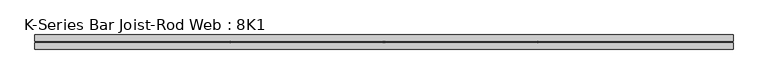
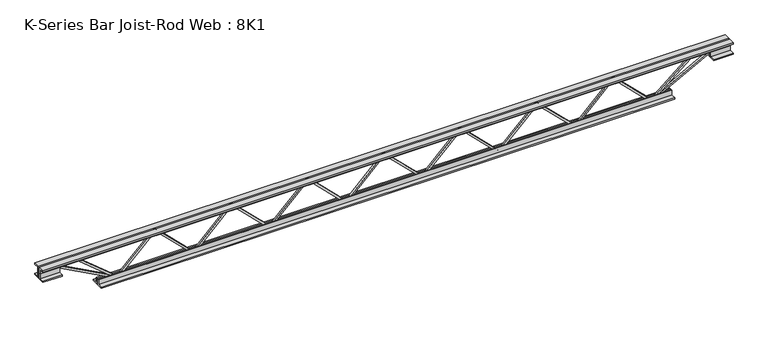
"""IFC4 building model written with IfcOpenShell, lengths in millimetres: beam geometry, K-Series Bar Joist-Rod Web : 8K1."""

from ifc_helpers import new_model, si_unit, frame, origin, place, context, project, spatial, polyline, outline, extrude, source, transform, mapped, element, save


def k_series_bar_joist_rod_web_8k1_41fa30a3(model_context):
    return source(origin(), model_context, "Body", "SweptSolid", [
        extrude(outline(polyline([(-90.4875, 598.572914), (-100.0125, 598.572914), (-100.0125, 603.7011887), (90.4875, 796.8754933), (90.4875, 799.3189439), (-100.0125, 992.4932486), (-100.0125, 997.6215233), (-90.4875, 997.6215233), (-90.4875, 996.399798), (100.0125, 803.2254933), (100.0125, 792.9689439), (-90.4875, 599.7946393), (-90.4875, 598.572914)])), frame((0.0, -4.7625, 0.0), z_axis=(0.0, 1.0, 0.0), x_axis=(0.0, 0.0, 1.0)), (0.0, 0.0, 1.0), 9.525),
        extrude(outline(polyline([(-90.4875, 199.5243047), (-100.0125, 199.5243047), (-100.0125, 204.6525794), (90.4875, 397.826884), (90.4875, 400.2703346), (-100.0125, 593.4446393), (-100.0125, 598.572914), (-90.4875, 598.572914), (-90.4875, 597.3511887), (100.0125, 404.176884), (100.0125, 393.9203346), (-90.4875, 200.74603), (-90.4875, 199.5243047)])), frame((0.0, -4.7625, 0.0), z_axis=(0.0, 1.0, 0.0), x_axis=(0.0, 0.0, 1.0)), (0.0, 0.0, 1.0), 9.525),
        extrude(outline(polyline([(-90.4875, -199.5243047), (-100.0125, -199.5243047), (-100.0125, -194.39603), (90.4875, -1.2217253), (90.4875, 1.2217253), (-100.0125, 194.39603), (-100.0125, 199.5243047), (-90.4875, 199.5243047), (-90.4875, 198.3025794), (100.0125, 5.1282747), (100.0125, -5.1282747), (-90.4875, -198.3025794), (-90.4875, -199.5243047)])), frame((0.0, -4.7625, 0.0), z_axis=(0.0, 1.0, 0.0), x_axis=(0.0, 0.0, 1.0)), (0.0, 0.0, 1.0), 9.525),
        extrude(outline(polyline([(-90.4875, -598.572914), (-100.0125, -598.572914), (-100.0125, -593.4446393), (90.4875, -400.2703346), (90.4875, -397.826884), (-100.0125, -204.6525794), (-100.0125, -199.5243047), (-90.4875, -199.5243047), (-90.4875, -200.74603), (100.0125, -393.9203346), (100.0125, -404.176884), (-90.4875, -597.3511887), (-90.4875, -598.572914)])), frame((0.0, -4.7625, 0.0), z_axis=(0.0, 1.0, 0.0), x_axis=(0.0, 0.0, 1.0)), (0.0, 0.0, 1.0), 9.525),
        extrude(outline(polyline([(-90.4875, -997.6215233), (-100.0125, -997.6215233), (-100.0125, -992.4932486), (90.4875, -799.3189439), (90.4875, -796.8754933), (-100.0125, -603.7011887), (-100.0125, -598.572914), (-90.4875, -598.572914), (-90.4875, -599.7946393), (100.0125, -792.9689439), (100.0125, -803.2254933), (-90.4875, -996.399798), (-90.4875, -997.6215233)])), frame((0.0, -4.7625, 0.0), z_axis=(0.0, 1.0, 0.0), x_axis=(0.0, 0.0, 1.0)), (0.0, 0.0, 1.0), 9.525),
        extrude(outline(polyline([(-90.4875, 997.6215233), (-100.0125, 997.6215233), (-100.0125, 1002.749798), (90.4875, 1195.9241027), (90.4875, 1198.3675532), (-100.0125, 1391.5418579), (-100.0125, 1396.6701326), (-90.4875, 1396.6701326), (-90.4875, 1395.4484073), (100.0125, 1202.2741027), (100.0125, 1192.0175532), (-90.4875, 998.8432486), (-90.4875, 997.6215233)])), frame((0.0, -4.7625, 0.0), z_axis=(0.0, 1.0, 0.0), x_axis=(0.0, 0.0, 1.0)), (0.0, 0.0, 1.0), 9.525),
        extrude(outline(polyline([(-90.4875, -1396.6701326), (-100.0125, -1396.6701326), (-100.0125, -1391.5418579), (90.4875, -1198.3675532), (90.4875, -1195.9241027), (-100.0125, -1002.749798), (-100.0125, -997.6215233), (-90.4875, -997.6215233), (-90.4875, -998.8432486), (100.0125, -1192.0175532), (100.0125, -1202.2741027), (-90.4875, -1395.4484073), (-90.4875, -1396.6701326)])), frame((0.0, -4.7625, 0.0), z_axis=(0.0, 1.0, 0.0), x_axis=(0.0, 0.0, 1.0)), (0.0, 0.0, 1.0), 9.525),
        extrude(outline(polyline([(4.7625, 101.6), (36.5125, 101.6), (36.5125, 95.25), (11.1125, 95.25), (11.1125, 69.85), (4.7625, 69.85), (4.7625, 101.6)])), frame((-1803.0701326, 0.0, 0.0), z_axis=(1.0, 0.0, 0.0), x_axis=(0.0, 1.0, 0.0)), (0.0, 0.0, 1.0), 3606.1402652),
        extrude(outline(polyline([(-4.7625, 101.6), (-4.7625, 69.85), (-11.1125, 69.85), (-11.1125, 95.25), (-36.5125, 95.25), (-36.5125, 101.6), (-4.7625, 101.6)])), frame((-1803.0701326, 0.0, 0.0), z_axis=(1.0, 0.0, 0.0), x_axis=(0.0, 1.0, 0.0)), (0.0, 0.0, 1.0), 3606.1402652),
        extrude(outline(polyline([(-4.7625, 38.1), (-36.5125, 38.1), (-36.5125, 44.45), (-11.1125, 44.45), (-11.1125, 69.85), (-4.7625, 69.85), (-4.7625, 38.1)])), frame((-1803.0701326, 0.0, 0.0), z_axis=(1.0, 0.0, 0.0), x_axis=(0.0, 1.0, 0.0)), (0.0, 0.0, 1.0), 101.6),
        extrude(outline(polyline([(36.5125, 38.1), (4.7625, 38.1), (4.7625, 69.85), (11.1125, 69.85), (11.1125, 44.45), (36.5125, 44.45), (36.5125, 38.1)])), frame((-1803.0701326, 0.0, 0.0), z_axis=(1.0, 0.0, 0.0), x_axis=(0.0, 1.0, 0.0)), (0.0, 0.0, 1.0), 101.6),
        extrude(outline(polyline([(4.7625, 38.1), (4.7625, 69.85), (11.1125, 69.85), (11.1125, 44.45), (36.5125, 44.45), (36.5125, 38.1), (4.7625, 38.1)])), frame((1701.4701326, 0.0, 0.0), z_axis=(1.0, 0.0, 0.0), x_axis=(0.0, 1.0, 0.0)), (0.0, 0.0, 1.0), 101.6),
        extrude(outline(polyline([(-4.7625, 38.1), (-36.5125, 38.1), (-36.5125, 44.45), (-11.1125, 44.45), (-11.1125, 69.85), (-4.7625, 69.85), (-4.7625, 38.1)])), frame((1701.4701326, 0.0, 0.0), z_axis=(1.0, 0.0, 0.0), x_axis=(0.0, 1.0, 0.0)), (0.0, 0.0, 1.0), 101.6),
        extrude(outline(polyline([(4.7625, -101.6), (4.7625, -69.85), (11.1125, -69.85), (11.1125, -95.25), (36.5125, -95.25), (36.5125, -101.6), (4.7625, -101.6)])), frame((-1498.2701326, 0.0, 0.0), z_axis=(1.0, 0.0, 0.0), x_axis=(0.0, 1.0, 0.0)), (0.0, 0.0, 1.0), 2996.5402652),
        extrude(outline(polyline([(-4.7625, -101.6), (-36.5125, -101.6), (-36.5125, -95.25), (-11.1125, -95.25), (-11.1125, -69.85), (-4.7625, -69.85), (-4.7625, -101.6)])), frame((-1498.2701326, 0.0, 0.0), z_axis=(1.0, 0.0, 0.0), x_axis=(0.0, 1.0, 0.0)), (0.0, 0.0, 1.0), 2996.5402652),
        extrude(outline(polyline([(0.0, -9.525), (0.0, 0.0), (346.6425392, 0.0), (346.6425392, -9.525), (0.0, -9.525)])), frame((-1703.7384311, 4.7625, 65.662372), z_axis=(0.4762831485400801, 0.0, 0.8792919665371384), x_axis=(0.8792919665371384, 0.0, -0.4762831485400801)), (0.0, 0.0, 1.0), 9.525),
        extrude(outline(polyline([(0.0, -9.525), (0.0, 0.0), (258.9748214, 0.0), (258.9748214, -9.525), (0.0, -9.525)])), frame((-1599.2305963, 4.7625, 66.1807842), z_axis=(0.6375137129935787, 0.0, 0.7704390084524154), x_axis=(0.7704390084524154, 0.0, -0.6375137129935787)), (0.0, 0.0, 1.0), 9.525),
        extrude(outline(polyline([(0.0, -9.525), (0.0, 0.0), (346.6425392, 0.0), (346.6425392, -9.525), (0.0, -9.525)])), frame((1703.7384311, -4.7625, 65.662372), z_axis=(-0.4762831485400428, 0.0, 0.8792919665371586), x_axis=(-0.8792919665371586, 0.0, -0.4762831485400428)), (0.0, 0.0, 1.0), 9.525),
        extrude(outline(polyline([(0.0, -9.525), (0.0, 0.0), (258.9748214, 0.0), (258.9748214, -9.525), (0.0, -9.525)])), frame((1599.2305963, -4.7625, 66.1807842), z_axis=(-0.6375137129935525, 0.0, 0.7704390084524371), x_axis=(-0.7704390084524371, 0.0, -0.6375137129935525)), (0.0, 0.0, 1.0), 9.525),
    ])


if __name__ == "__main__":
    model = new_model("IFC4")
    model_context = context("Model", 3, world=origin())
    ifc_project = project(units=[si_unit("LENGTHUNIT", "METRE", prefix="MILLI")], contexts=[model_context])
    site = spatial("IfcSite", under=ifc_project)
    building = spatial("IfcBuilding", under=site)
    placement = place(None, origin())
    k_series_bar_joist_rod_web_8k1_shape = k_series_bar_joist_rod_web_8k1_41fa30a3(model_context)
    element("IfcBeam", 1, ObjectType="K-Series Bar Joist-Rod Web : 8K1", at=placement, inside=building, context=model_context, shape_type="MappedRepresentation", body=[
        mapped(k_series_bar_joist_rod_web_8k1_shape, transform((0.0, 0.0, 0.0), x_axis=(1.0, 0.0, 0.0), y_axis=(0.0, 1.0, 0.0), z_axis=(0.0, 0.0, 1.0))),
    ])
    save(model, "model.ifc")

# Revit data of these elements
# Type "K-Series Bar Joist-Rod Web : 8K1"
#   Assembly Code = "B1010350"
#   Wt = 5.1
#   Web Thickness = 0' - 0 3/8"
#   Start Offset [instance default] = 0' - 0"
#   Start Extension [instance default] = 0' - 0"
#   Seat Length = 0' - 4"
#   Seat Depth = 0' - 2 1/2"
#   PanelArrayLength [instance default] = 21' - 4"
#   Panel [instance default] = 1' - 4"
#   End Offset [instance default] = 0' - 0"
#   End Extension [instance default] = 0' - 0"
#   End Panel = 1' - 4"
#   Cord Leg = 0' - 1 1/4"
#   Chord Thickness = 0' - 0 1/4"
#   Length [instance default] = 24' - 0"
#   Depth = 0' - 8"
#   PanelArrayNum [instance default] = 16
#   Rendering Material = none
# Element 1 (IfcBeam, "K-Series Bar Joist-Rod Web : 8K1")
#   PanelArrayLength = 9' - 1.97403"
#   Panel = 1' - 3.71058"
#   PanelArrayNum = 7
